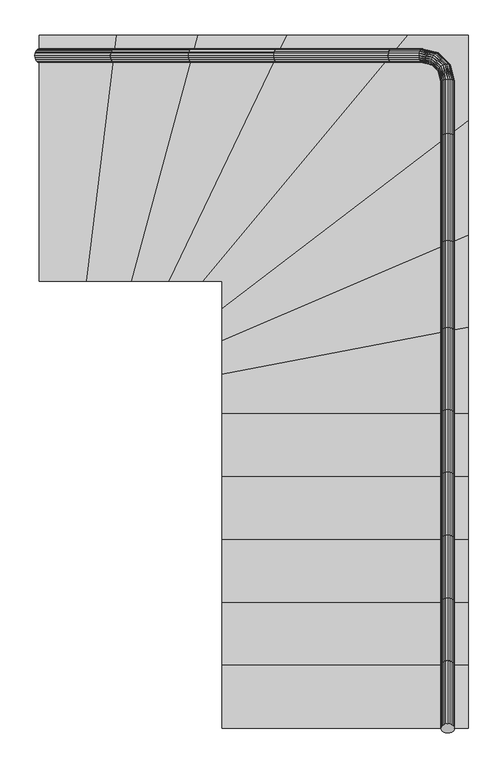
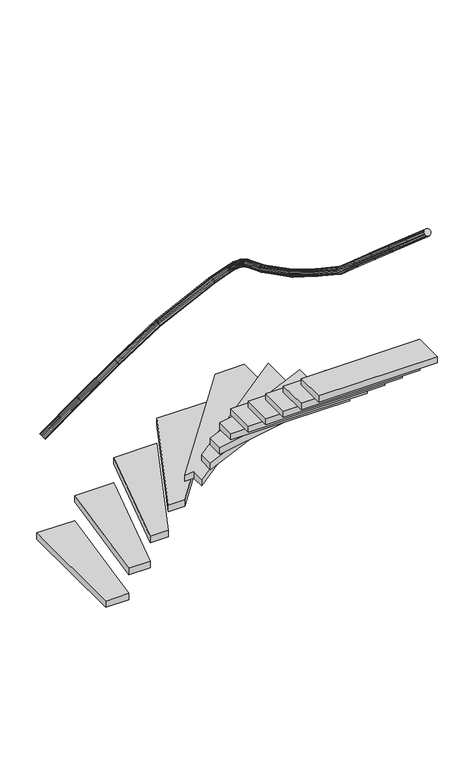
"""IFC4 building model written with IfcOpenShell, lengths in millimetres: stair geometry, 0_3d."""

from ifc_helpers import new_model, si_unit, frame, origin, origin_with_axes, place, context, project, spatial, polyline, outline, extrude, faceted_brep, source, transform, mapped, element, save


def stair_75b24629(model_context):
    return source(origin(), model_context, "Body", "SolidModel", [
        extrude(outline(polyline([(1.2235871, -7.9923213), (0.0, 0.0), (1.2235871, 7.9923214), (4.7745752, 15.2022986), (10.3053687, 20.9241691), (17.2745752, 24.5978359), (25.0, 25.8636953), (32.7254249, 24.5978359), (39.6946313, 20.9241691), (45.2254249, 15.2022986), (48.7764129, 7.9923214), (50.0, 0.0), (48.7764129, -7.9923213), (45.2254249, -15.2022986), (39.6946313, -20.924169), (32.7254249, -24.5978359), (25.0, -25.8636953), (17.2745752, -24.5978359), (10.3053687, -20.924169), (4.7745752, -15.2022986), (1.2235871, -7.9923213)])), frame((1485.1870834, 936.9712063, 2669.5592366), z_axis=(0.0, -0.7546055221634622, 0.6561787149248356), x_axis=(1.0, 0.0, 0.0)), (0.0, 0.0, 1.0), 304.7950131),
        faceted_brep([(890.7630529, 2452.79663, 1462.5710073), (886.853034, 2451.5730429, 1469.5592366), (882.9430152, 2452.79663, 1476.5474659), (879.4157362, 2456.3476181, 1482.8516386), (876.6164718, 2461.8784116, 1487.8546583), (874.8192334, 2468.8476181, 1491.0667948), (874.1999472, 2476.5730429, 1492.1736216), (874.8192334, 2484.2984678, 1491.0667948), (876.6164718, 2491.2676742, 1487.8546583), (879.4157362, 2496.7984678, 1482.8516386), (882.9430152, 2500.3494558, 1476.5474659), (886.853034, 2501.5730429, 1469.5592366), (890.7630529, 2500.3494558, 1462.5710073), (894.2903318, 2496.7984678, 1456.2668346), (897.0895963, 2491.2676742, 1451.2638149), (898.8868347, 2484.2984678, 1448.0516784), (899.5061208, 2476.5730429, 1446.9448517), (898.8868347, 2468.8476181, 1448.0516784), (897.0895963, 2461.8784116, 1451.2638149), (894.2903318, 2456.3476181, 1456.2668346), (1299.6991056, 2452.79663, 1676.8834604), (1302.9101599, 2451.5730429, 1669.5592366), (1306.1212141, 2452.79663, 1662.2350128), (1309.017948, 2456.3476181, 1655.627735), (1311.316809, 2461.8784116, 1650.3841697), (1312.7927686, 2468.8476181, 1647.0175936), (1313.3013497, 2476.5730429, 1645.8575505), (1312.7927686, 2484.2984678, 1647.0175936), (1311.316809, 2491.2676742, 1650.3841697), (1309.017948, 2496.7984678, 1655.627735), (1306.1212141, 2500.3494558, 1662.2350128), (1302.9101599, 2501.5730429, 1669.5592366), (1299.6991056, 2500.3494558, 1676.8834604), (1296.8023718, 2496.7984678, 1683.4907382), (1294.5035107, 2491.2676742, 1688.7343035), (1293.0275511, 2484.2984678, 1692.1008796), (1292.5189701, 2476.5730429, 1693.2609227), (1293.0275511, 2468.8476181, 1692.1008796), (1294.5035107, 2461.8784116, 1688.7343035), (1296.8023718, 2456.3476181, 1683.4907382)], [[[0, 1, 2, 3, 4, 5, 6, 7, 8, 9, 10, 11, 12, 13, 14, 15, 16, 17, 18, 19]], [[20, 21, 22, 23, 24, 25, 26, 27, 28, 29, 30, 31, 32, 33, 34, 35, 36, 37, 38, 39]], [[2, 1, 21, 20]], [[3, 2, 20, 39]], [[4, 3, 39, 38]], [[5, 4, 38, 37]], [[6, 5, 37, 36]], [[7, 6, 36, 35]], [[8, 7, 35, 34]], [[9, 8, 34, 33]], [[10, 9, 33, 32]], [[11, 10, 32, 31]], [[12, 11, 31, 30]], [[13, 12, 30, 29]], [[14, 13, 29, 28]], [[15, 14, 28, 27]], [[16, 15, 27, 26]], [[17, 16, 26, 25]], [[18, 17, 25, 24]], [[19, 18, 24, 23]], [[0, 19, 23, 22]], [[1, 0, 22, 21]]]),
        extrude(outline(polyline([(1585.1870834, 1483.1289049), (1585.1870834, 1166.9712063), (685.1870834, 1166.9712063), (685.1870834, 1310.8135078), (1585.1870834, 1483.1289049)])), frame((0.0, 0.0, 1400.0), z_axis=(0.0, 0.0, 1.0), x_axis=(1.0, 0.0, 0.0)), (0.0, 0.0, 1.0), 50.0),
        extrude(outline(polyline([(1585.1870834, 1819.7779009), (1585.1870834, 1483.1289049), (685.1870834, 1310.8135078), (685.1870834, 1434.6945611), (1585.1870834, 1819.7779009)])), frame((0.0, 0.0, 1200.0), z_axis=(0.0, 0.0, 1.0), x_axis=(1.0, 0.0, 0.0)), (0.0, 0.0, 1.0), 50.0),
        extrude(outline(polyline([(1365.4304396, 2551.5730429), (1585.1870834, 2551.5730429), (1585.1870834, 2237.7659758), (685.1870834, 1551.5730429), (685.1870834, 1651.5730429), (615.1870834, 1651.5730429), (1365.4304396, 2551.5730429)])), frame((0.0, 0.0, 800.0), z_axis=(0.0, 0.0, 1.0), x_axis=(1.0, 0.0, 0.0)), (0.0, 0.0, 1.0), 50.0),
        faceted_brep([(1486.4106705, 1783.7438024, 2062.5985679), (1485.1870834, 1787.6876226, 2069.5592366), (1486.4106705, 1791.6314427, 2076.5199053), (1489.9616586, 1795.1892143, 2082.7992152), (1495.4924521, 1798.0126778, 2087.7825038), (1502.4616586, 1799.8254529, 2090.981972), (1510.1870834, 1800.4500927, 2092.0844336), (1517.9125083, 1799.8254529, 2090.981972), (1524.8817147, 1798.0126778, 2087.7825038), (1530.4125083, 1795.1892143, 2082.7992152), (1533.9634963, 1791.6314427, 2076.5199053), (1535.1870834, 1787.6876226, 2069.5592366), (1533.9634963, 1783.7438024, 2062.5985679), (1530.4125083, 1780.1860309, 2056.319258), (1524.8817147, 1777.3625674, 2051.3359694), (1517.9125083, 1775.5497922, 2048.1365012), (1510.1870834, 1774.9251525, 2047.0340396), (1502.4616586, 1775.5497922, 2048.1365012), (1495.4924521, 1777.3625674, 2051.3359694), (1489.9616586, 1780.1860309, 2056.319258), (1486.4106705, 1473.100594, 2276.2769055), (1485.1870834, 1468.7692885, 2269.5592366), (1486.4106705, 1464.4379829, 2262.8415677), (1489.9616586, 1460.5306557, 2256.781471), (1495.4924521, 1457.4297833, 2251.9721511), (1502.4616586, 1455.4389007, 2248.8843776), (1510.1870834, 1454.7528893, 2247.8204034), (1517.9125083, 1455.4389007, 2248.8843776), (1524.8817147, 1457.4297833, 2251.9721511), (1530.4125083, 1460.5306557, 2256.781471), (1533.9634963, 1464.4379829, 2262.8415677), (1535.1870834, 1468.7692885, 2269.5592366), (1533.9634963, 1473.100594, 2276.2769055), (1530.4125083, 1477.0079212, 2282.3370022), (1524.8817147, 1480.1087936, 2287.1463221), (1517.9125083, 1482.0996763, 2290.2340956), (1510.1870834, 1482.7856877, 2291.2980698), (1502.4616586, 1482.0996763, 2290.2340956), (1495.4924521, 1480.1087936, 2287.1463221), (1489.9616586, 1477.0079212, 2282.3370022)], [[[0, 1, 2, 3, 4, 5, 6, 7, 8, 9, 10, 11, 12, 13, 14, 15, 16, 17, 18, 19]], [[20, 21, 22, 23, 24, 25, 26, 27, 28, 29, 30, 31, 32, 33, 34, 35, 36, 37, 38, 39]], [[2, 1, 21, 20]], [[3, 2, 20, 39]], [[4, 3, 39, 38]], [[5, 4, 38, 37]], [[6, 5, 37, 36]], [[7, 6, 36, 35]], [[8, 7, 35, 34]], [[9, 8, 34, 33]], [[10, 9, 33, 32]], [[11, 10, 32, 31]], [[12, 11, 31, 30]], [[13, 12, 30, 29]], [[14, 13, 29, 28]], [[15, 14, 28, 27]], [[16, 15, 27, 26]], [[17, 16, 26, 25]], [[18, 17, 25, 24]], [[19, 18, 24, 23]], [[0, 19, 23, 22]], [[1, 0, 22, 21]]]),
        extrude(outline(polyline([(922.7634492, 2551.5730429), (1365.4304396, 2551.5730429), (615.1870834, 1651.5730429), (491.8384675, 1651.5730429), (922.7634492, 2551.5730429)])), frame((0.0, 0.0, 600.0), z_axis=(0.0, 0.0, 1.0), x_axis=(1.0, 0.0, 0.0)), (0.0, 0.0, 1.0), 50.0),
        extrude(outline(polyline([(1585.1870834, 706.9712063), (1585.1870834, 476.9712063), (685.1870834, 476.9712063), (685.1870834, 706.9712063), (1585.1870834, 706.9712063)])), frame((0.0, 0.0, 2000.0), z_axis=(0.0, 0.0, 1.0), x_axis=(1.0, 0.0, 0.0)), (0.0, 0.0, 1.0), 50.0),
        faceted_brep([(1486.4106705, 1464.4379829, 2262.8415677), (1485.1870834, 1468.7692885, 2269.5592366), (1486.4106705, 1473.100594, 2276.2769055), (1489.9616586, 1477.0079212, 2282.3370022), (1495.4924521, 1480.1087936, 2287.1463221), (1502.4616586, 1482.0996763, 2290.2340956), (1510.1870834, 1482.7856877, 2291.2980698), (1517.9125083, 1482.0996763, 2290.2340956), (1524.8817147, 1480.1087936, 2287.1463221), (1530.4125083, 1477.0079212, 2282.3370022), (1533.9634963, 1473.100594, 2276.2769055), (1535.1870834, 1468.7692885, 2269.5592366), (1533.9634963, 1464.4379829, 2262.8415677), (1530.4125083, 1460.5306557, 2256.781471), (1524.8817147, 1457.4297833, 2251.9721511), (1517.9125083, 1455.4389007, 2248.8843776), (1510.1870834, 1454.7528893, 2247.8204034), (1502.4616586, 1455.4389007, 2248.8843776), (1495.4924521, 1457.4297833, 2251.9721511), (1489.9616586, 1460.5306557, 2256.781471), (1486.4106705, 1171.8215247, 2475.9329585), (1485.1870834, 1166.9712063, 2469.5592366), (1486.4106705, 1162.120888, 2463.1855148), (1489.9616586, 1157.7453526, 2457.4356972), (1495.4924521, 1154.272908, 2452.8726162), (1502.4616586, 1152.0434614, 2449.9429378), (1510.1870834, 1151.2752464, 2448.9334394), (1517.9125083, 1152.0434614, 2449.9429378), (1524.8817147, 1154.272908, 2452.8726162), (1530.4125083, 1157.7453526, 2457.4356972), (1533.9634963, 1162.120888, 2463.1855148), (1535.1870834, 1166.9712063, 2469.5592366), (1533.9634963, 1171.8215247, 2475.9329585), (1530.4125083, 1176.1970601, 2481.682776), (1524.8817147, 1179.6695046, 2486.2458571), (1517.9125083, 1181.8989513, 2489.1755354), (1510.1870834, 1182.6671663, 2490.1850338), (1502.4616586, 1181.8989513, 2489.1755354), (1495.4924521, 1179.6695046, 2486.2458571), (1489.9616586, 1176.1970601, 2481.682776)], [[[0, 1, 2, 3, 4, 5, 6, 7, 8, 9, 10, 11, 12, 13, 14, 15, 16, 17, 18, 19]], [[20, 21, 22, 23, 24, 25, 26, 27, 28, 29, 30, 31, 32, 33, 34, 35, 36, 37, 38, 39]], [[2, 1, 21, 20]], [[3, 2, 20, 39]], [[4, 3, 39, 38]], [[5, 4, 38, 37]], [[6, 5, 37, 36]], [[7, 6, 36, 35]], [[8, 7, 35, 34]], [[9, 8, 34, 33]], [[10, 9, 33, 32]], [[11, 10, 32, 31]], [[12, 11, 31, 30]], [[13, 12, 30, 29]], [[14, 13, 29, 28]], [[15, 14, 28, 27]], [[16, 15, 27, 26]], [[17, 16, 26, 25]], [[18, 17, 25, 24]], [[19, 18, 24, 23]], [[0, 19, 23, 22]], [[1, 0, 22, 21]]]),
        extrude(outline(polyline([(1585.1870834, 1166.9712063), (1585.1870834, 936.9712063), (685.1870834, 936.9712063), (685.1870834, 1166.9712063), (1585.1870834, 1166.9712063)])), frame((0.0, 0.0, 1600.0), z_axis=(0.0, 0.0, 1.0), x_axis=(1.0, 0.0, 0.0)), (0.0, 0.0, 1.0), 50.0),
        extrude(outline(polyline([(1.2235871, -7.9923213), (0.0, 0.0), (1.2235871, 7.9923214), (4.7745752, 15.2022986), (10.3053687, 20.9241691), (17.2745752, 24.5978359), (25.0, 25.8636953), (32.7254249, 24.5978359), (39.6946313, 20.9241691), (45.2254249, 15.2022986), (48.7764129, 7.9923214), (50.0, 0.0), (48.7764129, -7.9923213), (45.2254249, -15.2022986), (39.6946313, -20.924169), (32.7254249, -24.5978359), (25.0, -25.8636953), (17.2745752, -24.5978359), (10.3053687, -20.924169), (4.7745752, -15.2022986), (1.2235871, -7.9923213)])), frame((1485.1870834, 246.9712063, 3269.5592366), z_axis=(0.0, -0.7546055221634872, 0.6561787149248068), x_axis=(1.0, 0.0, 0.0)), (0.0, 0.0, 1.0), 304.7950131),
        extrude(outline(polyline([(1585.1870834, 936.9712063), (1585.1870834, 706.9712063), (685.1870834, 706.9712063), (685.1870834, 936.9712063), (1585.1870834, 936.9712063)])), frame((0.0, 0.0, 1800.0), z_axis=(0.0, 0.0, 1.0), x_axis=(1.0, 0.0, 0.0)), (0.0, 0.0, 1.0), 50.0),
        extrude(outline(polyline([(596.5161775, 2551.5730429), (922.7634492, 2551.5730429), (491.8384675, 1651.5730429), (353.8579893, 1651.5730429), (596.5161775, 2551.5730429)])), frame((0.0, 0.0, 400.0), z_axis=(0.0, 0.0, 1.0), x_axis=(1.0, 0.0, 0.0)), (0.0, 0.0, 1.0), 50.0),
        extrude(outline(polyline([(1.2235871, -7.9923213), (0.0, 0.0), (1.2235871, 7.9923214), (4.7745752, 15.2022986), (10.3053687, 20.9241691), (17.2745752, 24.5978359), (25.0, 25.8636953), (32.7254249, 24.5978359), (39.6946313, 20.9241691), (45.2254249, 15.2022986), (48.7764129, 7.9923214), (50.0, 0.0), (48.7764129, -7.9923213), (45.2254249, -15.2022986), (39.6946313, -20.924169), (32.7254249, -24.5978359), (25.0, -25.8636953), (17.2745752, -24.5978359), (10.3053687, -20.924169), (4.7745752, -15.2022986), (1.2235871, -7.9923213)])), frame((1485.1870834, 706.9712063, 2869.5592366), z_axis=(0.0, -0.7546055221634878, 0.6561787149248063), x_axis=(1.0, 0.0, 0.0)), (0.0, 0.0, 1.0), 304.7950131),
        faceted_brep([(580.7533244, 2452.79663, 1262.9243346), (576.2946618, 2451.5730429, 1269.5592366), (571.8359993, 2452.79663, 1276.1941386), (567.8137816, 2456.3476181, 1282.1795702), (564.6217317, 2461.8784116, 1286.9296355), (562.5723094, 2468.8476181, 1289.9793652), (561.8661266, 2476.5730429, 1291.0302305), (562.5723094, 2484.2984678, 1289.9793652), (564.6217317, 2491.2676742, 1286.9296355), (567.8137816, 2496.7984678, 1282.1795702), (571.8359993, 2500.3494558, 1276.1941386), (576.2946618, 2501.5730429, 1269.5592366), (580.7533244, 2500.3494558, 1262.9243346), (584.775542, 2496.7984678, 1256.9389031), (587.967592, 2491.2676742, 1252.1888377), (590.0170142, 2484.2984678, 1249.139108), (590.723197, 2476.5730429, 1248.0882427), (590.0170142, 2468.8476181, 1249.139108), (587.967592, 2461.8784116, 1252.1888377), (584.775542, 2456.3476181, 1256.9389031), (882.9430152, 2452.79663, 1476.5474659), (886.853034, 2451.5730429, 1469.5592366), (890.7630529, 2452.79663, 1462.5710073), (894.2903318, 2456.3476181, 1456.2668346), (897.0895963, 2461.8784116, 1451.2638149), (898.8868347, 2468.8476181, 1448.0516784), (899.5061208, 2476.5730429, 1446.9448517), (898.8868347, 2484.2984678, 1448.0516784), (897.0895963, 2491.2676742, 1451.2638149), (894.2903318, 2496.7984678, 1456.2668346), (890.7630529, 2500.3494558, 1462.5710073), (886.853034, 2501.5730429, 1469.5592366), (882.9430152, 2500.3494558, 1476.5474659), (879.4157362, 2496.7984678, 1482.8516386), (876.6164718, 2491.2676742, 1487.8546583), (874.8192334, 2484.2984678, 1491.0667948), (874.1999472, 2476.5730429, 1492.1736216), (874.8192334, 2468.8476181, 1491.0667948), (876.6164718, 2461.8784116, 1487.8546583), (879.4157362, 2456.3476181, 1482.8516386)], [[[0, 1, 2, 3, 4, 5, 6, 7, 8, 9, 10, 11, 12, 13, 14, 15, 16, 17, 18, 19]], [[20, 21, 22, 23, 24, 25, 26, 27, 28, 29, 30, 31, 32, 33, 34, 35, 36, 37, 38, 39]], [[2, 1, 21, 20]], [[3, 2, 20, 39]], [[4, 3, 39, 38]], [[5, 4, 38, 37]], [[6, 5, 37, 36]], [[7, 6, 36, 35]], [[8, 7, 35, 34]], [[9, 8, 34, 33]], [[10, 9, 33, 32]], [[11, 10, 32, 31]], [[12, 11, 31, 30]], [[13, 12, 30, 29]], [[14, 13, 29, 28]], [[15, 14, 28, 27]], [[16, 15, 27, 26]], [[17, 16, 26, 25]], [[18, 17, 25, 24]], [[19, 18, 24, 23]], [[0, 19, 23, 22]], [[1, 0, 22, 21]]]),
        extrude(outline(polyline([(15.1870834, 2551.5730429), (300.0242482, 2551.5730429), (190.3499186, 1651.5730429), (15.1870834, 1651.5730429), (15.1870834, 2551.5730429)])), origin_with_axes(), (0.0, 0.0, 1.0), 50.0),
        faceted_brep([(1486.4106705, 1162.120888, 2463.1855148), (1485.1870834, 1166.9712063, 2469.5592366), (1486.4106705, 1171.8215247, 2475.9329585), (1489.9616586, 1176.1970601, 2481.682776), (1495.4924521, 1179.6695046, 2486.2458571), (1502.4616586, 1181.8989513, 2489.1755354), (1510.1870834, 1182.6671663, 2490.1850338), (1517.9125083, 1181.8989513, 2489.1755354), (1524.8817147, 1179.6695046, 2486.2458571), (1530.4125083, 1176.1970601, 2481.682776), (1533.9634963, 1171.8215247, 2475.9329585), (1535.1870834, 1166.9712063, 2469.5592366), (1533.9634963, 1162.120888, 2463.1855148), (1530.4125083, 1157.7453526, 2457.4356972), (1524.8817147, 1154.272908, 2452.8726162), (1517.9125083, 1152.0434614, 2449.9429378), (1510.1870834, 1151.2752464, 2448.9334394), (1502.4616586, 1152.0434614, 2449.9429378), (1495.4924521, 1154.272908, 2452.8726162), (1489.9616586, 1157.7453526, 2457.4356972), (1486.4106705, 942.2155975, 2675.5902865), (1485.1870834, 936.9712063, 2669.5592366), (1486.4106705, 931.7268152, 2663.5281868), (1489.9616586, 926.9957815, 2658.0874981), (1495.4924521, 923.241212, 2653.7697431), (1502.4616586, 920.83063, 2650.9975738), (1510.1870834, 920.0, 2650.0423493), (1517.9125083, 920.83063, 2650.9975738), (1524.8817147, 923.241212, 2653.7697431), (1530.4125083, 926.9957815, 2658.0874981), (1533.9634963, 931.7268152, 2663.5281868), (1535.1870834, 936.9712063, 2669.5592366), (1533.9634963, 942.2155975, 2675.5902865), (1530.4125083, 946.9466311, 2681.0309751), (1524.8817147, 950.7012007, 2685.3487301), (1517.9125083, 953.1117827, 2688.1208994), (1510.1870834, 953.9424127, 2689.0761239), (1502.4616586, 953.1117827, 2688.1208994), (1495.4924521, 950.7012007, 2685.3487301), (1489.9616586, 946.9466311, 2681.0309751)], [[[0, 1, 2, 3, 4, 5, 6, 7, 8, 9, 10, 11, 12, 13, 14, 15, 16, 17, 18, 19]], [[20, 21, 22, 23, 24, 25, 26, 27, 28, 29, 30, 31, 32, 33, 34, 35, 36, 37, 38, 39]], [[2, 1, 21, 20]], [[3, 2, 20, 39]], [[4, 3, 39, 38]], [[5, 4, 38, 37]], [[6, 5, 37, 36]], [[7, 6, 36, 35]], [[8, 7, 35, 34]], [[9, 8, 34, 33]], [[10, 9, 33, 32]], [[11, 10, 32, 31]], [[12, 11, 31, 30]], [[13, 12, 30, 29]], [[14, 13, 29, 28]], [[15, 14, 28, 27]], [[16, 15, 27, 26]], [[17, 16, 26, 25]], [[18, 17, 25, 24]], [[19, 18, 24, 23]], [[0, 19, 23, 22]], [[1, 0, 22, 21]]]),
        faceted_brep([(19.8801503, 2452.79663, 863.0898994), (15.1870834, 2451.5730429, 869.5592366), (10.4940165, 2452.79663, 876.0285738), (6.2603398, 2456.3476181, 881.8646473), (2.9004748, 2461.8784116, 886.4961814), (0.7433088, 2468.8476181, 889.4698093), (0.0, 2476.5730429, 890.4944517), (0.7433088, 2484.2984678, 889.4698093), (2.9004748, 2491.2676742, 886.4961814), (6.2603398, 2496.7984678, 881.8646473), (10.4940165, 2500.3494558, 876.0285738), (15.1870834, 2501.5730429, 869.5592366), (19.8801503, 2500.3494558, 863.0898994), (24.1138271, 2496.7984678, 857.2538259), (27.473692, 2491.2676742, 852.6222918), (29.6308581, 2484.2984678, 849.6486639), (30.3741668, 2476.5730429, 848.6240215), (29.6308581, 2468.8476181, 849.6486639), (27.473692, 2461.8784116, 852.6222918), (24.1138271, 2456.3476181, 857.2538259), (286.2445898, 2452.79663, 1076.0669753), (290.8847207, 2451.5730429, 1069.5592366), (295.5248517, 2452.79663, 1063.0514979), (299.7107743, 2456.3476181, 1057.1807821), (303.0327413, 2461.8784116, 1052.5217556), (305.1655754, 2468.8476181, 1049.5304765), (305.9004999, 2476.5730429, 1048.4997519), (305.1655754, 2484.2984678, 1049.5304765), (303.0327413, 2491.2676742, 1052.5217556), (299.7107743, 2496.7984678, 1057.1807821), (295.5248517, 2500.3494558, 1063.0514979), (290.8847207, 2501.5730429, 1069.5592366), (286.2445898, 2500.3494558, 1076.0669753), (282.0586672, 2496.7984678, 1081.9376911), (278.7367002, 2491.2676742, 1086.5967176), (276.6038661, 2484.2984678, 1089.5879968), (275.8689415, 2476.5730429, 1090.6187213), (276.6038661, 2468.8476181, 1089.5879968), (278.7367002, 2461.8784116, 1086.5967176), (282.0586672, 2456.3476181, 1081.9376911)], [[[0, 1, 2, 3, 4, 5, 6, 7, 8, 9, 10, 11, 12, 13, 14, 15, 16, 17, 18, 19]], [[20, 21, 22, 23, 24, 25, 26, 27, 28, 29, 30, 31, 32, 33, 34, 35, 36, 37, 38, 39]], [[2, 1, 21, 20]], [[3, 2, 20, 39]], [[4, 3, 39, 38]], [[5, 4, 38, 37]], [[6, 5, 37, 36]], [[7, 6, 36, 35]], [[8, 7, 35, 34]], [[9, 8, 34, 33]], [[10, 9, 33, 32]], [[11, 10, 32, 31]], [[12, 11, 31, 30]], [[13, 12, 30, 29]], [[14, 13, 29, 28]], [[15, 14, 28, 27]], [[16, 15, 27, 26]], [[17, 16, 26, 25]], [[18, 17, 25, 24]], [[19, 18, 24, 23]], [[0, 19, 23, 22]], [[1, 0, 22, 21]]]),
        extrude(outline(polyline([(1.2235871, -7.9923213), (0.0, 0.0), (1.2235871, 7.9923214), (4.7745752, 15.2022986), (10.3053687, 20.9241691), (17.2745752, 24.5978359), (25.0, 25.8636953), (32.7254249, 24.5978359), (39.6946313, 20.9241691), (45.2254249, 15.2022986), (48.7764129, 7.9923214), (50.0, 0.0), (48.7764129, -7.9923213), (45.2254249, -15.2022986), (39.6946313, -20.924169), (32.7254249, -24.5978359), (25.0, -25.8636953), (17.2745752, -24.5978359), (10.3053687, -20.924169), (4.7745752, -15.2022986), (1.2235871, -7.9923213)])), frame((1485.1870834, 476.9712063, 3069.5592366), z_axis=(0.0, -0.754605522163459, 0.6561787149248393), x_axis=(1.0, 0.0, 0.0)), (0.0, 0.0, 1.0), 304.7950131),
        extrude(outline(polyline([(300.0242482, 2551.5730429), (596.5161775, 2551.5730429), (353.8579893, 1651.5730429), (190.3499186, 1651.5730429), (300.0242482, 2551.5730429)])), frame((0.0, 0.0, 200.0), z_axis=(0.0, 0.0, 1.0), x_axis=(1.0, 0.0, 0.0)), (0.0, 0.0, 1.0), 50.0),
        extrude(outline(polyline([(1585.1870834, 2237.7659758), (1585.1870834, 1819.7779009), (685.1870834, 1434.6945611), (685.1870834, 1551.5730429), (1585.1870834, 2237.7659758)])), frame((0.0, 0.0, 1000.0), z_axis=(0.0, 0.0, 1.0), x_axis=(1.0, 0.0, 0.0)), (0.0, 0.0, 1.0), 50.0),
        faceted_brep([(295.5248517, 2452.79663, 1063.0514979), (290.8847207, 2451.5730429, 1069.5592366), (286.2445898, 2452.79663, 1076.0669753), (282.0586672, 2456.3476181, 1081.9376911), (278.7367002, 2461.8784116, 1086.5967176), (276.6038661, 2468.8476181, 1089.5879968), (275.8689415, 2476.5730429, 1090.6187213), (276.6038661, 2484.2984678, 1089.5879968), (278.7367002, 2491.2676742, 1086.5967176), (282.0586672, 2496.7984678, 1081.9376911), (286.2445898, 2500.3494558, 1076.0669753), (290.8847207, 2501.5730429, 1069.5592366), (295.5248517, 2500.3494558, 1063.0514979), (299.7107743, 2496.7984678, 1057.1807821), (303.0327413, 2491.2676742, 1052.5217556), (305.1655754, 2484.2984678, 1049.5304765), (305.9004999, 2476.5730429, 1048.4997519), (305.1655754, 2468.8476181, 1049.5304765), (303.0327413, 2461.8784116, 1052.5217556), (299.7107743, 2456.3476181, 1057.1807821), (571.8359993, 2452.79663, 1276.1941386), (576.2946618, 2451.5730429, 1269.5592366), (580.7533244, 2452.79663, 1262.9243346), (584.775542, 2456.3476181, 1256.9389031), (587.967592, 2461.8784116, 1252.1888377), (590.0170142, 2468.8476181, 1249.139108), (590.723197, 2476.5730429, 1248.0882427), (590.0170142, 2484.2984678, 1249.139108), (587.967592, 2491.2676742, 1252.1888377), (584.775542, 2496.7984678, 1256.9389031), (580.7533244, 2500.3494558, 1262.9243346), (576.2946618, 2501.5730429, 1269.5592366), (571.8359993, 2500.3494558, 1276.1941386), (567.8137816, 2496.7984678, 1282.1795702), (564.6217317, 2491.2676742, 1286.9296355), (562.5723094, 2484.2984678, 1289.9793652), (561.8661266, 2476.5730429, 1291.0302305), (562.5723094, 2468.8476181, 1289.9793652), (564.6217317, 2461.8784116, 1286.9296355), (567.8137816, 2456.3476181, 1282.1795702)], [[[0, 1, 2, 3, 4, 5, 6, 7, 8, 9, 10, 11, 12, 13, 14, 15, 16, 17, 18, 19]], [[20, 21, 22, 23, 24, 25, 26, 27, 28, 29, 30, 31, 32, 33, 34, 35, 36, 37, 38, 39]], [[2, 1, 21, 20]], [[3, 2, 20, 39]], [[4, 3, 39, 38]], [[5, 4, 38, 37]], [[6, 5, 37, 36]], [[7, 6, 36, 35]], [[8, 7, 35, 34]], [[9, 8, 34, 33]], [[10, 9, 33, 32]], [[11, 10, 32, 31]], [[12, 11, 31, 30]], [[13, 12, 30, 29]], [[14, 13, 29, 28]], [[15, 14, 28, 27]], [[16, 15, 27, 26]], [[17, 16, 26, 25]], [[18, 17, 25, 24]], [[19, 18, 24, 23]], [[0, 19, 23, 22]], [[1, 0, 22, 21]]]),
        faceted_brep([(1486.4106705, 2177.2875031, 1862.2686626), (1485.1870834, 2180.5832314, 1869.5592366), (1486.4106705, 2183.8789598, 1876.8498106), (1489.9616586, 2186.8520793, 1883.4267324), (1495.4924521, 2189.2115603, 1888.6462072), (1502.4616586, 2190.7264404, 1891.9973162), (1510.1870834, 2191.2484324, 1893.1520297), (1517.9125083, 2190.7264404, 1891.9973162), (1524.8817147, 2189.2115603, 1888.6462072), (1530.4125083, 2186.8520793, 1883.4267324), (1533.9634963, 2183.8789598, 1876.8498106), (1535.1870834, 2180.5832314, 1869.5592366), (1533.9634963, 2177.2875031, 1862.2686626), (1530.4125083, 2174.3143835, 1855.6917408), (1524.8817147, 2171.9549025, 1850.4722661), (1517.9125083, 2170.4400225, 1847.121157), (1510.1870834, 2169.9180304, 1845.9664435), (1502.4616586, 2170.4400225, 1847.121157), (1495.4924521, 2171.9549025, 1850.4722661), (1489.9616586, 2174.3143835, 1855.6917408), (1486.4106705, 1791.6314427, 2076.5199053), (1485.1870834, 1787.6876226, 2069.5592366), (1486.4106705, 1783.7438024, 2062.5985679), (1489.9616586, 1780.1860309, 2056.319258), (1495.4924521, 1777.3625674, 2051.3359694), (1502.4616586, 1775.5497922, 2048.1365012), (1510.1870834, 1774.9251525, 2047.0340396), (1517.9125083, 1775.5497922, 2048.1365012), (1524.8817147, 1777.3625674, 2051.3359694), (1530.4125083, 1780.1860309, 2056.319258), (1533.9634963, 1783.7438024, 2062.5985679), (1535.1870834, 1787.6876226, 2069.5592366), (1533.9634963, 1791.6314427, 2076.5199053), (1530.4125083, 1795.1892143, 2082.7992152), (1524.8817147, 1798.0126778, 2087.7825038), (1517.9125083, 1799.8254529, 2090.981972), (1510.1870834, 1800.4500927, 2092.0844336), (1502.4616586, 1799.8254529, 2090.981972), (1495.4924521, 1798.0126778, 2087.7825038), (1489.9616586, 1795.1892143, 2082.7992152)], [[[0, 1, 2, 3, 4, 5, 6, 7, 8, 9, 10, 11, 12, 13, 14, 15, 16, 17, 18, 19]], [[20, 21, 22, 23, 24, 25, 26, 27, 28, 29, 30, 31, 32, 33, 34, 35, 36, 37, 38, 39]], [[2, 1, 21, 20]], [[3, 2, 20, 39]], [[4, 3, 39, 38]], [[5, 4, 38, 37]], [[6, 5, 37, 36]], [[7, 6, 36, 35]], [[8, 7, 35, 34]], [[9, 8, 34, 33]], [[10, 9, 33, 32]], [[11, 10, 32, 31]], [[12, 11, 31, 30]], [[13, 12, 30, 29]], [[14, 13, 29, 28]], [[15, 14, 28, 27]], [[16, 15, 27, 26]], [[17, 16, 26, 25]], [[18, 17, 25, 24]], [[19, 18, 24, 23]], [[0, 19, 23, 22]], [[1, 0, 22, 21]]]),
        extrude(outline(polyline([(1585.1870834, 476.9712063), (1585.1870834, 246.9712063), (685.1870834, 246.9712063), (685.1870834, 476.9712063), (1585.1870834, 476.9712063)])), frame((0.0, 0.0, 2200.0), z_axis=(0.0, 0.0, 1.0), x_axis=(1.0, 0.0, 0.0)), (0.0, 0.0, 1.0), 50.0),
        extrude(outline(polyline([(1585.1870834, 246.9712063), (1585.1870834, 16.9712063), (685.1870834, 16.9712063), (685.1870834, 246.9712063), (1585.1870834, 246.9712063)])), frame((0.0, 0.0, 2400.0), z_axis=(0.0, 0.0, 1.0), x_axis=(1.0, 0.0, 0.0)), (0.0, 0.0, 1.0), 50.0),
        faceted_brep([(1306.1212141, 2452.79663, 1662.2350128), (1302.9101599, 2451.5730429, 1669.5592366), (1299.6991056, 2452.79663, 1676.8834604), (1296.8023718, 2456.3476181, 1683.4907382), (1294.5035107, 2461.8784116, 1688.7343035), (1293.0275511, 2468.8476181, 1692.1008796), (1292.5189701, 2476.5730429, 1693.2609227), (1293.0275511, 2484.2984678, 1692.1008796), (1294.5035107, 2491.2676742, 1688.7343035), (1296.8023718, 2496.7984678, 1683.4907382), (1299.6991056, 2500.3494558, 1676.8834604), (1302.9101599, 2501.5730429, 1669.5592366), (1306.1212141, 2500.3494558, 1662.2350128), (1309.017948, 2496.7984678, 1655.627735), (1311.316809, 2491.2676742, 1650.3841697), (1312.7927686, 2484.2984678, 1647.0175936), (1313.3013497, 2476.5730429, 1645.8575505), (1312.7927686, 2468.8476181, 1647.0175936), (1311.316809, 2461.8784116, 1650.3841697), (1309.017948, 2456.3476181, 1655.627735), (1486.4106705, 2183.8789598, 1876.8498106), (1485.1870834, 2180.5832314, 1869.5592366), (1486.4106705, 2177.2875031, 1862.2686626), (1489.9616586, 2174.3143835, 1855.6917408), (1495.4924521, 2171.9549025, 1850.4722661), (1502.4616586, 2170.4400225, 1847.121157), (1510.1870834, 2169.9180304, 1845.9664435), (1517.9125083, 2170.4400225, 1847.121157), (1524.8817147, 2171.9549025, 1850.4722661), (1530.4125083, 2174.3143835, 1855.6917408), (1533.9634963, 2177.2875031, 1862.2686626), (1535.1870834, 2180.5832314, 1869.5592366), (1533.9634963, 2183.8789598, 1876.8498106), (1530.4125083, 2186.8520793, 1883.4267324), (1524.8817147, 2189.2115603, 1888.6462072), (1517.9125083, 2190.7264404, 1891.9973162), (1510.1870834, 2191.2484324, 1893.1520297), (1502.4616586, 2190.7264404, 1891.9973162), (1495.4924521, 2189.2115603, 1888.6462072), (1489.9616586, 2186.8520793, 1883.4267324), (1414.0458947, 2451.5730429, 1713.724975), (1411.094253, 2452.79663, 1721.1522903), (1408.4315386, 2456.3476181, 1727.8525682), (1406.3183965, 2461.8784116, 1733.1699389), (1404.9616757, 2468.8476181, 1736.583901), (1404.4941816, 2476.5730429, 1737.7602722), (1404.9616757, 2484.2984678, 1736.583901), (1406.3183965, 2491.2676742, 1733.1699389), (1408.4315386, 2496.7984678, 1727.8525682), (1411.094253, 2500.3494558, 1721.1522903), (1414.0458947, 2501.5730429, 1713.724975), (1416.9975363, 2500.3494558, 1706.2976597), (1419.6602507, 2496.7984678, 1699.5973818), (1421.7733928, 2491.2676742, 1694.2800111), (1423.1301136, 2484.2984678, 1690.866049), (1423.5976077, 2476.5730429, 1689.6896778), (1423.1301136, 2468.8476181, 1690.866049), (1421.7733928, 2461.8784116, 1694.2800111), (1419.6602507, 2456.3476181, 1699.5973818), (1416.9975363, 2452.79663, 1706.2976597), (1452.7287908, 2442.604699, 1738.6559048), (1449.9885418, 2445.5007167, 1745.6899991), (1448.6921205, 2450.2595609, 1752.0355473), (1448.9664298, 2456.4154029, 1757.0714029), (1450.7846183, 2463.365666, 1760.3046212), (1453.9687091, 2470.43001, 1761.4187123), (1458.2070211, 2476.9169277, 1760.3046212), (1463.084679, 2482.1914344, 1757.0714029), (1468.1242235, 2485.7372245, 1752.0355473), (1472.8323489, 2487.2072116, 1745.6899991), (1476.748191, 2486.457503, 1738.6559048), (1479.4884401, 2483.5614853, 1731.6218104), (1480.7848614, 2478.8026411, 1725.2762623), (1480.5105521, 2472.6467991, 1720.2404067), (1478.6923636, 2465.696536, 1717.0071884), (1475.5082728, 2458.632192, 1715.8930973), (1471.2699607, 2452.1452743, 1717.0071884), (1466.3923029, 2446.8707676, 1720.2404067), (1461.3527584, 2443.3249774, 1725.2762623), (1456.644633, 2441.8549904, 1731.6218104), (1476.2187395, 2419.1147504, 1765.2077495), (1475.4690309, 2423.0305925, 1772.2418439), (1476.9390179, 2427.7387179, 1778.5873921), (1480.4848081, 2432.7782624, 1783.6232476), (1485.7593148, 2437.6559202, 1786.8564659), (1492.2462325, 2441.8942323, 1787.970557), (1499.3105765, 2445.0783231, 1786.8564659), (1506.2608396, 2446.8965116, 1783.6232476), (1512.4166816, 2447.1708209, 1778.5873921), (1517.1755258, 2445.8743996, 1772.2418439), (1520.0715435, 2443.1341506, 1765.2077495), (1520.8212521, 2439.2183084, 1758.1736552), (1519.351265, 2434.510183, 1751.828107), (1515.8054748, 2429.4706385, 1746.7922515), (1510.5309682, 2424.5929807, 1743.5590332), (1504.0440505, 2420.3546686, 1742.4449421), (1496.9797065, 2417.1705778, 1743.5590332), (1490.0294434, 2415.3523893, 1746.7922515), (1483.8736014, 2415.07808, 1751.828107), (1479.1147571, 2416.3745013, 1758.1736552), (1485.1870834, 2380.4318542, 1790.1386793), (1486.4106705, 2383.3834958, 1797.5659946), (1489.9616586, 2386.0462102, 1804.2662726), (1495.4924521, 2388.1593524, 1809.5836432), (1502.4616586, 2389.5160731, 1812.9976054), (1510.1870834, 2389.9835672, 1814.1739765), (1517.9125083, 2389.5160731, 1812.9976054), (1524.8817147, 2388.1593524, 1809.5836432), (1530.4125083, 2386.0462102, 1804.2662726), (1533.9634963, 2383.3834958, 1797.5659946), (1535.1870834, 2380.4318542, 1790.1386793), (1533.9634963, 2377.4802125, 1782.711364), (1530.4125083, 2374.8174981, 1776.0110861), (1524.8817147, 2372.704356, 1770.6937155), (1517.9125083, 2371.3476352, 1767.2797533), (1510.1870834, 2370.8801411, 1766.1033822), (1502.4616586, 2371.3476352, 1767.2797533), (1495.4924521, 2372.704356, 1770.6937155), (1489.9616586, 2374.8174981, 1776.0110861), (1486.4106705, 2377.4802125, 1782.711364)], [[[0, 1, 2, 3, 4, 5, 6, 7, 8, 9, 10, 11, 12, 13, 14, 15, 16, 17, 18, 19]], [[20, 21, 22, 23, 24, 25, 26, 27, 28, 29, 30, 31, 32, 33, 34, 35, 36, 37, 38, 39]], [[2, 1, 40, 41]], [[3, 2, 41, 42]], [[4, 3, 42, 43]], [[5, 4, 43, 44]], [[6, 5, 44, 45]], [[7, 6, 45, 46]], [[8, 7, 46, 47]], [[9, 8, 47, 48]], [[10, 9, 48, 49]], [[11, 10, 49, 50]], [[12, 11, 50, 51]], [[13, 12, 51, 52]], [[14, 13, 52, 53]], [[15, 14, 53, 54]], [[16, 15, 54, 55]], [[17, 16, 55, 56]], [[18, 17, 56, 57]], [[19, 18, 57, 58]], [[0, 19, 58, 59]], [[1, 0, 59, 40]], [[41, 40, 60]], [[61, 41, 60]], [[42, 41, 61]], [[62, 42, 61]], [[43, 42, 62]], [[63, 43, 62]], [[44, 43, 63]], [[64, 44, 63]], [[45, 44, 64]], [[65, 45, 64]], [[46, 45, 65]], [[66, 46, 65]], [[47, 46, 66]], [[67, 47, 66]], [[48, 47, 67]], [[68, 48, 67]], [[49, 48, 68]], [[69, 49, 68]], [[50, 49, 69]], [[70, 50, 69]], [[51, 50, 70]], [[71, 51, 70]], [[52, 51, 71]], [[72, 52, 71]], [[53, 52, 72]], [[73, 53, 72]], [[54, 53, 73]], [[74, 54, 73]], [[55, 54, 74]], [[75, 55, 74]], [[56, 55, 75]], [[76, 56, 75]], [[57, 56, 76]], [[77, 57, 76]], [[58, 57, 77]], [[78, 58, 77]], [[59, 58, 78]], [[79, 59, 78]], [[40, 59, 79]], [[60, 40, 79]], [[61, 60, 80]], [[81, 61, 80]], [[62, 61, 81]], [[82, 62, 81]], [[63, 62, 82]], [[83, 63, 82]], [[64, 63, 83]], [[84, 64, 83]], [[65, 64, 84]], [[85, 65, 84]], [[66, 65, 85]], [[86, 66, 85]], [[67, 66, 86]], [[87, 67, 86]], [[68, 67, 87]], [[88, 68, 87]], [[69, 68, 88]], [[89, 69, 88]], [[70, 69, 89]], [[90, 70, 89]], [[71, 70, 90]], [[91, 71, 90]], [[72, 71, 91]], [[92, 72, 91]], [[73, 72, 92]], [[93, 73, 92]], [[74, 73, 93]], [[94, 74, 93]], [[75, 74, 94]], [[95, 75, 94]], [[76, 75, 95]], [[96, 76, 95]], [[77, 76, 96]], [[97, 77, 96]], [[78, 77, 97]], [[98, 78, 97]], [[79, 78, 98]], [[99, 79, 98]], [[60, 79, 99]], [[80, 60, 99]], [[81, 80, 100]], [[101, 81, 100]], [[82, 81, 101]], [[102, 82, 101]], [[83, 82, 102]], [[103, 83, 102]], [[84, 83, 103]], [[104, 84, 103]], [[85, 84, 104]], [[105, 85, 104]], [[86, 85, 105]], [[106, 86, 105]], [[87, 86, 106]], [[107, 87, 106]], [[88, 87, 107]], [[108, 88, 107]], [[89, 88, 108]], [[109, 89, 108]], [[90, 89, 109]], [[110, 90, 109]], [[91, 90, 110]], [[111, 91, 110]], [[92, 91, 111]], [[112, 92, 111]], [[93, 92, 112]], [[113, 93, 112]], [[94, 93, 113]], [[114, 94, 113]], [[95, 94, 114]], [[115, 95, 114]], [[96, 95, 115]], [[116, 96, 115]], [[97, 96, 116]], [[117, 97, 116]], [[98, 97, 117]], [[118, 98, 117]], [[99, 98, 118]], [[119, 99, 118]], [[80, 99, 119]], [[100, 80, 119]], [[101, 100, 21, 20]], [[102, 101, 20, 39]], [[103, 102, 39, 38]], [[104, 103, 38, 37]], [[105, 104, 37, 36]], [[106, 105, 36, 35]], [[107, 106, 35, 34]], [[108, 107, 34, 33]], [[109, 108, 33, 32]], [[110, 109, 32, 31]], [[111, 110, 31, 30]], [[112, 111, 30, 29]], [[113, 112, 29, 28]], [[114, 113, 28, 27]], [[115, 114, 27, 26]], [[116, 115, 26, 25]], [[117, 116, 25, 24]], [[118, 117, 24, 23]], [[119, 118, 23, 22]], [[100, 119, 22, 21]]]),
    ])


if __name__ == "__main__":
    model = new_model("IFC4")
    model_context = context("Model", 3, world=origin())
    ifc_project = project(units=[si_unit("LENGTHUNIT", "METRE", prefix="MILLI")], contexts=[model_context])
    site = spatial("IfcSite", under=ifc_project)
    building = spatial("IfcBuilding", under=site)
    placement = place(None, origin())
    stair_shape = stair_75b24629(model_context)
    element("IfcStair", 1, ObjectType="0_3d", at=placement, inside=building, context=model_context, shape_type="MappedRepresentation", body=[
        mapped(stair_shape, transform((0.0, 0.0, 0.0), x_axis=(1.0, 0.0, 0.0), y_axis=(0.0, 1.0, 0.0), z_axis=(0.0, 0.0, 1.0))),
    ])
    save(model, "model.ifc")

# Revit data of these elements
# Element 1 (IfcStair, "0_3d")
#   Materials on its faces: "*1", "weiss"
# Materials
#   "*1": class "Unassigned", colour RGB 175 175 175, transparency 0
#   "weiss": class "Unassigned", colour RGB 255 255 255, transparency 0
